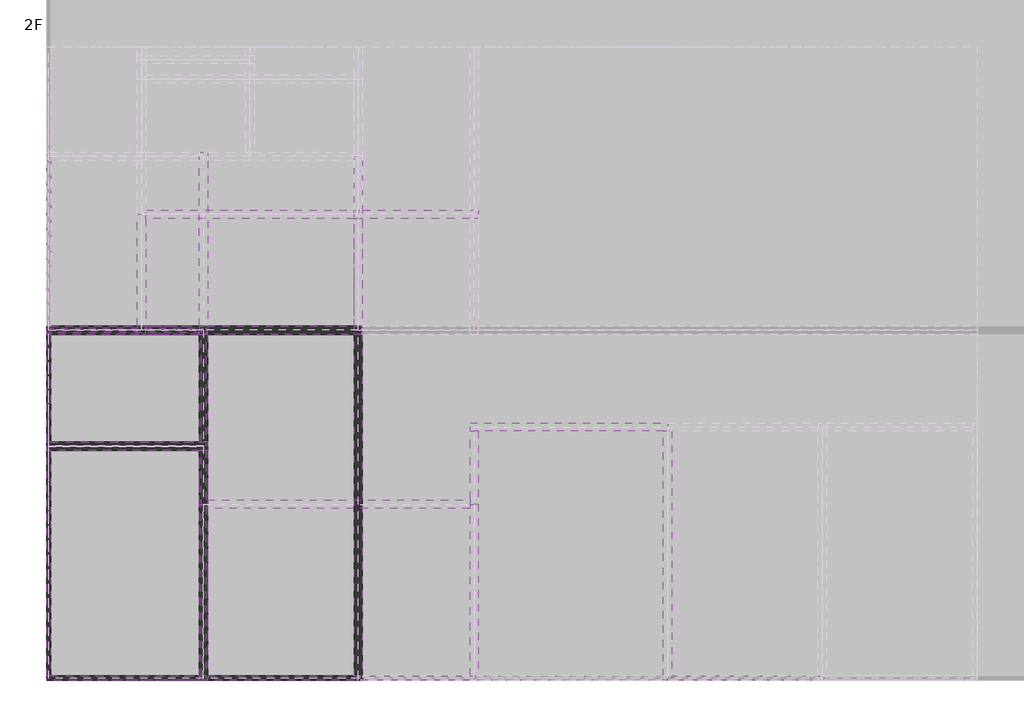
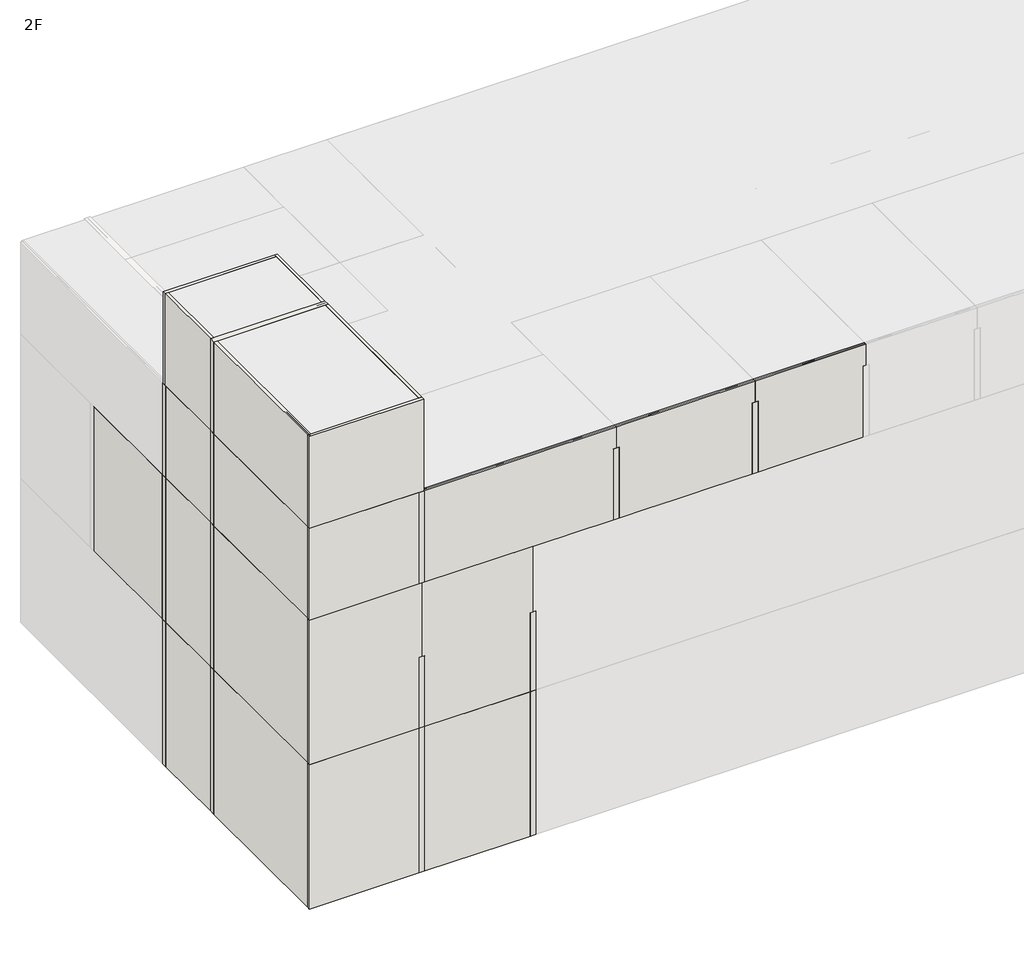
# One storey, part 1 of 3: 51 walls.
# Revit data of these elements (continued)
# Room at (70459.652, 168423.861) mm, phase "New Construction", upper offset 5500 mm, lower offset 0 mm (continued)
#   Floor Finish = "FL1"
#   Number = "2.1"
#   Name = "Electrical Room-2"
#   Interior Finish = "IW5..N/A..N/A,,WK1..N/A,,FL1..N/A,,CL1..N/A"
#   Exterior Finish = "N/A..N/A,,EW1..EW2..N/A"
# Room at (82459.652, 177423.861) mm, phase "New Construction", upper offset 5500 mm, lower offset 0 mm
#   Department = "AR"
#   Base Finish = "WK1"
#   Ceiling Finish = "CL1"
#   Wall Finish = "IW5"
#   Floor Finish = "FL1"
#   Number = "2.2"
#   Name = "Electrical Room (GIS)"
#   Interior Finish = "IW5..N/A..N/A,,WK1..N/A,,FL1..N/A,,CL1..N/A"
#   Exterior Finish = "N/A..N/A,,EW1..EW2..N/A"
# Room at (51459.652, 168423.861) mm, phase "New Construction", upper offset 2700 mm, lower offset 0 mm
#   Department = "AR"
#   Base Finish = "WK3"
#   Ceiling Finish = "CL3"
#   Wall Finish = "IW5"
#   Floor Finish = "FL2"
#   Number = "2.3"
#   Name = "Lobby"
#   Interior Finish = "IW5..N/A..N/A,,WK3..N/A,,FL2..N/A,,CL3..N/A"
#   Exterior Finish = "N/A..N/A,,EW2..N/A..N/A"
# Room at (47459.652, 171423.861) mm, phase "New Construction", upper offset 5500 mm, lower offset 0 mm
#   Department = "PATHV2"
#   Base Finish = ""
#   Ceiling Finish = ""
#   Wall Finish = ""
#   Floor Finish = ""
#   Number = "2.4"
#   Name = "Elevator"
#   Interior Finish = "N/A..N/A..N/A,,N/A..N/A,,N/A..N/A,,N/A..N/A"
#   Exterior Finish = "N/A..N/A,,EW2..N/A..N/A"
# Room at (47459.652, 166923.861) mm, phase "New Construction", upper offset 5500 mm, lower offset 0 mm
#   Department = "PATHV1"
#   Base Finish = "WK3"
#   Ceiling Finish = "CL1"
#   Wall Finish = "IW5"
#   Floor Finish = "FL2"
#   Number = "2.5"
#   Name = "Staircase"
#   Interior Finish = "IW5..N/A..N/A,,WK3..N/A,,FL2..N/A,,CL1..N/A"
#   Exterior Finish = "N/A..N/A,,EW2..N/A..N/A"
# Room at (65459.652, 177423.861) mm, phase "New Construction", upper offset 3400 mm, lower offset 0 mm
#   Department = "CI"
#   Base Finish = ""
#   Ceiling Finish = "CL3"
#   Wall Finish = "IW5"
#   Floor Finish = "FL5"
#   Number = "3.0"
#   Name = "Central Control Room"
#   Interior Finish = "IW5..N/A..N/A,,N/A..N/A,,FL5..N/A,,CL3..N/A"
#   Exterior Finish = "N/A..N/A,,EW1..N/A..N/A"
# Room at (65459.652, 168423.861) mm, phase "New Construction", upper offset 3000 mm, lower offset 0 mm
#   Department = "CI"
#   Base Finish = ""
#   Ceiling Finish = "CL3"
#   Wall Finish = "IW5"
#   Floor Finish = "FL5"
#   Number = "3.1"
#   Name = "Electronic Room"
#   Interior Finish = "IW5..N/A..N/A,,N/A..N/A,,FL5..N/A,,CL3..N/A"
#   Exterior Finish = "N/A..N/A,,EW1..N/A..N/A"
# Room at (80959.652, 180173.861) mm, phase "New Construction", upper offset 2700 mm, lower offset 0 mm
#   Department = "AR"
#   Base Finish = ""
#   Ceiling Finish = "CL3"
#   Wall Finish = "IW5"
#   Floor Finish = "FL5"
#   Number = "3.2"
#   Name = "Computer Room"
#   Interior Finish = "IW5..N/A..N/A,,N/A..N/A,,FL5..N/A,,CL3..N/A"
#   Exterior Finish = "N/A..N/A,,EW2..N/A..N/A"
# Room at (82459.652, 168423.861) mm, phase "New Construction", upper offset 5500 mm, lower offset 0 mm
#   Department = "EL"
#   Base Finish = ""
#   Ceiling Finish = "CL3"
#   Wall Finish = "IW5"
#   Floor Finish = "FL5"
#   Number = "3.3"
#   Name = "Electrical Room -3"
#   Interior Finish = "IW5..N/A..N/A,,N/A..N/A,,FL5,,CL3..N/A"
#   Exterior Finish = "N/A..N/A,,EW2..N/A..N/A"
# Room at (80959.652, 174673.861) mm, phase "New Construction", upper offset 2700 mm, lower offset 0 mm
#   Department = "CI"
#   Base Finish = ""
#   Ceiling Finish = "CL3"
#   Wall Finish = "IW5"
#   Floor Finish = "FL5"
#   Number = "3.4"
#   Name = "Communication Room"
#   Interior Finish = "IW5..N/A..N/A,,N/A..N/A,,FL5..N/A,,CL3..N/A"
#   Exterior Finish = "N/A..N/A,,N/A..N/A..N/A"
# Room at (46659.652, 179673.861) mm, phase "New Construction", upper offset 5500 mm, lower offset 0 mm
#   Department = "PATHV3"
#   Base Finish = ""
#   Ceiling Finish = ""
#   Wall Finish = ""
#   Floor Finish = ""
#   Number = "3.5"
#   Name = "Duct Shaft"
#   Interior Finish = "N/A..N/A..N/A,,N/A..N/A,,N/A..N/A,,N/A..N/A"
#   Exterior Finish = "N/A..N/A,,EW2..N/A..N/A"
# Room at (47459.652, 175173.861) mm, phase "New Construction", upper offset 2700 mm, lower offset 0 mm
#   Department = "AR"
#   Base Finish = ""
#   Ceiling Finish = "CL4"
#   Wall Finish = "IW3"
#   Floor Finish = "FL3"
#   Number = "3.6"
#   Name = "Toilet (M)"
#   Interior Finish = "IW3..N/A..N/A,,N/A..N/A,,FL3..N/A,,CL4..N/A"
#   Exterior Finish = "N/A..N/A,,EW2..N/A..N/A"
# Room at (52059.652, 179673.861) mm, phase "New Construction", upper offset 2700 mm, lower offset 0 mm
#   Department = "AR"
#   Base Finish = ""
#   Ceiling Finish = "CL4"
#   Wall Finish = "IW3"
#   Floor Finish = "FL3"
#   Number = "3.7"
#   Name = "Toilet"
#   Interior Finish = "IW3..N/A..N/A,,N/A..N/A,,FL3..N/A,,CL4..N/A"
#   Exterior Finish = "N/A..N/A,,EW2..N/A..N/A"
# Room at (49259.652, 180923.861) mm, phase "New Construction", upper offset 2700 mm, lower offset 0 mm
#   Department = "AR"
#   Base Finish = ""
#   Ceiling Finish = "CL4"
#   Wall Finish = "IW3"
#   Floor Finish = "FL3"
#   Number = "3.8"
#   Name = "Shower"
#   Interior Finish = "IW3..N/A..N/A,,N/A..N/A,,FL3..N/A,,CL4..N/A"
#   Exterior Finish = "N/A..N/A,,EW2..N/A..N/A"
# Room at (49259.652, 178673.861) mm, phase "New Construction", upper offset 2700 mm, lower offset 0 mm
#   Department = "AR"
#   Base Finish = "WK3"
#   Ceiling Finish = "CL3"
#   Wall Finish = "IW5"
#   Floor Finish = "FL2"
#   Number = "3.9"
#   Name = "Locker(F)"
#   Interior Finish = "IW5..N/A..N/A,,WK3..N/A,,FL2..N/A,,CL3..N/A"
#   Exterior Finish = "N/A..N/A,,N/A..N/A..N/A"
# Room at (47459.652, 171423.861) mm, phase "New Construction", upper offset 5500 mm, lower offset 0 mm
#   Department = "PATHV2"
#   Base Finish = ""
#   Ceiling Finish = ""
#   Wall Finish = ""
#   Floor Finish = ""
#   Number = "3.10"
#   Name = "Elevator"
#   Interior Finish = "N/A..N/A..N/A,,N/A..N/A,,N/A..N/A,,N/A..N/A"
#   Exterior Finish = "N/A..N/A,,EW2..N/A..N/A"
# Room at (47459.652, 166923.861) mm, phase "New Construction", upper offset 2700 mm, lower offset 0 mm
#   Department = "PATHV1"
#   Base Finish = "WK3"
#   Ceiling Finish = "CL1"
#   Wall Finish = "IW5"
#   Floor Finish = "FL2"
#   Number = "3.11"
#   Name = "Staircase"
#   Interior Finish = "IW5..N/A..N/A,,WK3..N/A,,FL2..N/A,,CL1..N/A"
#   Exterior Finish = "N/A..N/A,,EW2..N/A..N/A"
# Room at (82459.652, 177423.861) mm, phase "New Construction", upper offset 2700 mm, lower offset 0 mm
#   Department = "AR"
#   Base Finish = "WK3"
#   Ceiling Finish = "CL3"
#   Wall Finish = "IW5"
#   Floor Finish = "FL2"
#   Number = "3.12"
#   Name = "Corridor"
#   Interior Finish = "IW5..N/A..N/A,,WK3..N/A,,FL2..N/A,,CL3..N/A"
#   Exterior Finish = "N/A..N/A,,EW2..N/A..N/A"
# Room at (51459.652, 170673.861) mm, phase "New Construction", upper offset 2700 mm, lower offset 0 mm
#   Department = "AR"
#   Base Finish = "WK3"
#   Ceiling Finish = "CL3"
#   Wall Finish = "IW5"
#   Floor Finish = "FL2"
#   Number = "3.13"
#   Name = "Corridor"
#   Interior Finish = "IW5..N/A..N/A,,WK3..N/A,,FL2..N/A,,CL3..N/A"
#   Exterior Finish = "N/A..N/A,,EW2..N/A..N/A"
# Room at (63459.652, 167173.861) mm, phase "New Construction", upper offset 2700 mm, lower offset 0 mm
#   Department = "AR"
#   Base Finish = "WK3"
#   Ceiling Finish = "CL3"
#   Wall Finish = "IW5"
#   Floor Finish = "FL2"
#   Number = "4.0"
#   Name = "Manager Office-1"
#   Interior Finish = "IW5..N/A..N/A,,WK3..N/A,,FL2..N/A,,CL3..N/A"
#   Exterior Finish = "RF1..N/A,,EW1..N/A..N/A"
# Room at (67459.652, 167173.861) mm, phase "New Construction", upper offset 2700 mm, lower offset 0 mm
#   Department = "AR"
#   Base Finish = "WK3"
#   Ceiling Finish = "CL3"
#   Wall Finish = "IW5"
#   Floor Finish = "FL2"
#   Number = "4.1"
#   Name = "Manager Office-2"
#   Interior Finish = "IW5..N/A..N/A,,WK3..N/A,,FL2..N/A,,CL3..N/A"
#   Exterior Finish = "RF1..N/A,,EW1..N/A..N/A"
# Room at (78709.652, 178923.861) mm, phase "New Construction", upper offset 2700 mm, lower offset 0 mm
#   Department = "AR"
#   Base Finish = "WK3"
#   Ceiling Finish = "CL3"
#   Wall Finish = "IW5"
#   Floor Finish = "FL2"
#   Number = "4.2"
#   Name = "Meeting Room-1"
#   Interior Finish = "IW5..N/A..N/A,,WK3..N/A,,FL2..N/A,,CL3..N/A"
#   Exterior Finish = "RF1..N/A,,EW1..EW2..N/A"
# Room at (73459.652, 167173.861) mm, phase "New Construction", upper offset 2700 mm, lower offset 0 mm
#   Department = "AR"
#   Base Finish = "WK3"
#   Ceiling Finish = "CL3"
#   Wall Finish = "IW5"
#   Floor Finish = "FL2"
#   Number = "4.3"
#   Name = "Meeting Room-2"
#   Interior Finish = "IW5..N/A..N/A,,WK3..N/A,,FL2..N/A,,CL3..N/A"
#   Exterior Finish = "RF1..N/A,,EW1..N/A..N/A"
# Room at (64709.652, 177423.861) mm, phase "New Construction", upper offset 2700 mm, lower offset 0 mm
#   Department = "HV"
#   Base Finish = "WK3"
#   Ceiling Finish = "CL3"
#   Wall Finish = "IW5"
#   Floor Finish = "FL2"
#   Number = "4.4"
#   Name = "Open Office"
#   Interior Finish = "IW5..N/A..N/A,,WK3..N/A,,FL2..N/A,,CL3..N/A"
#   Exterior Finish = "RF1..N/A,,EW1..N/A..N/A"
# Room at (54959.652, 178923.861) mm, phase "New Construction", upper offset 2700 mm, lower offset 0 mm
#   Department = "AR"
#   Base Finish = "WK3"
#   Ceiling Finish = "CL3"
#   Wall Finish = "IW5"
#   Floor Finish = "FL2"
#   Number = "4.12"
#   Name = "Locker(M)"
#   Interior Finish = "IW5..N/A..N/A,,WK3..N/A,,FL2..N/A,,CL3..N/A"
#   Exterior Finish = "RF1..N/A,,EW1..N/A..N/A"
# Room at (50659.652, 174423.861) mm, phase "New Construction", upper offset 2700 mm, lower offset 0 mm
#   Department = "AR"
#   Base Finish = ""
#   Ceiling Finish = "CL4"
#   Wall Finish = "IW3"
#   Floor Finish = "FL3"
#   Number = "4.13"
#   Name = "Toilet(F)"
#   Interior Finish = "IW3..N/A..N/A,,N/A..N/A,,FL3..N/A,,CL4..N/A"
#   Exterior Finish = "RF1..N/A,,N/A..N/A..N/A"
# Room at (46659.652, 177423.861) mm, phase "New Construction", upper offset 3500 mm, lower offset 0 mm
#   Department = "PATHV3"
#   Base Finish = ""
#   Ceiling Finish = ""
#   Wall Finish = ""
#   Floor Finish = ""
#   Number = "4.14"
#   Name = "Duct Shaft"
#   Interior Finish = "N/A..N/A..N/A,,N/A..N/A,,N/A..N/A,,N/A..N/A"
#   Exterior Finish = "RF1..N/A,,EW2..N/A..N/A"
# Room at (47459.652, 171423.861) mm, phase "New Construction", upper offset 3500 mm, lower offset 0 mm
#   Department = "PATHV2"
#   Base Finish = ""
#   Ceiling Finish = ""
#   Wall Finish = ""
#   Floor Finish = ""
#   Number = "4.15"
#   Name = "Elevator"
#   Interior Finish = "N/A..N/A..N/A,,N/A..N/A,,N/A..N/A,,N/A..N/A"
#   Exterior Finish = "N/A..N/A,,EW2..N/A..N/A"
# Room at (47459.652, 166923.861) mm, phase "New Construction", upper offset 3500 mm, lower offset 0 mm
#   Department = "PATHV1"
#   Base Finish = ""
#   Ceiling Finish = "CL1"
#   Wall Finish = "IW5"
#   Floor Finish = "FL2"
#   Number = "4.16"
#   Name = "Staircase"
#   Interior Finish = "IW5..N/A..N/A,,N/A..N/A,,FL2..N/A,,CL1..N/A"
#   Exterior Finish = "N/A..N/A,,EW2..N/A..N/A"
# Room at (61397.694, 171673.861) mm, phase "New Construction", upper offset 2700 mm, lower offset 0 mm
#   Department = "AR"
#   Base Finish = "WK3"
#   Ceiling Finish = "CL3"
#   Wall Finish = "IW5"
#   Floor Finish = "FL2"
#   Number = "4.17"
#   Name = "Corridor"
#   Interior Finish = "IW5..N/A..N/A,,WK3..N/A,,FL2..N/A,,CL3..N/A"
#   Exterior Finish = "RF1..N/A,,EW2..N/A..N/A"
# Room at (47459.652, 171423.861) mm, phase "New Construction", upper offset 3500 mm, lower offset 0 mm
#   Department = "PATHV2"
#   Base Finish = ""
#   Ceiling Finish = ""
#   Wall Finish = ""
#   Floor Finish = ""
#   Number = "5.0"
#   Name = "Elevator"
#   Interior Finish = "N/A..N/A..N/A,,N/A..N/A,,N/A..N/A,,N/A..N/A"
#   Exterior Finish = "RF1..N/A,,EW2..EW1..N/A"
# Room at (47459.652, 166923.861) mm, phase "New Construction", upper offset 3500 mm, lower offset 0 mm
#   Department = "PATHV1"
#   Base Finish = "WK3"
#   Ceiling Finish = "CL1"
#   Wall Finish = "IW5"
#   Floor Finish = "FL2"
#   Number = "5.1"
#   Name = "Staircase"
#   Interior Finish = "IW5..N/A..N/A,,WK3..N/A,,FL2..N/A,,CL1..N/A"
#   Exterior Finish = "RF1..N/A,,EW2..EW1..N/A"
